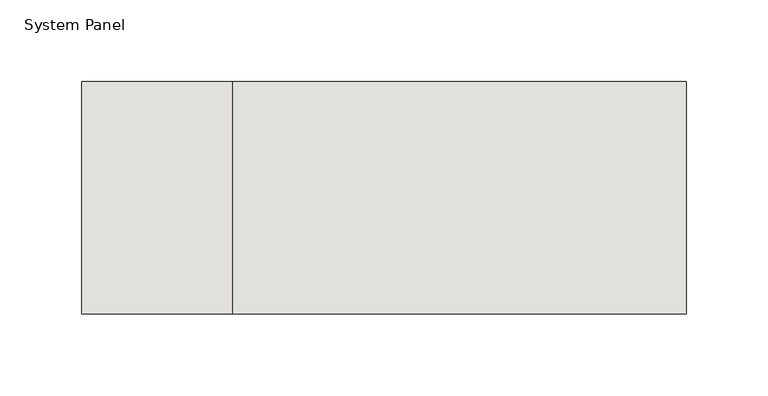
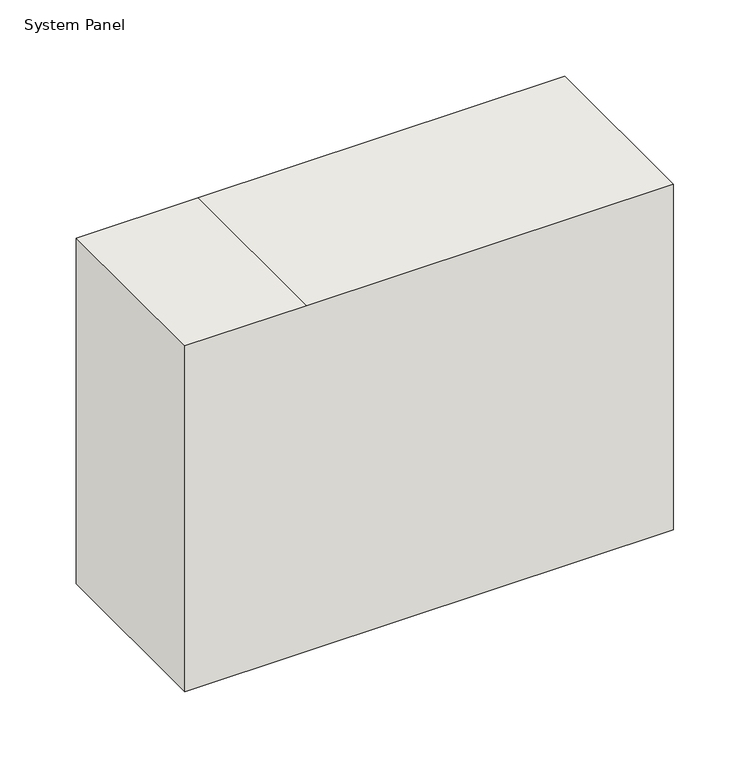
"""IFC4 building model written with IfcOpenShell, lengths in millimetres: wall geometry, System Panel : NLRS_21_CWP_hsb-vulling minerale wol 142 _gen_rsf."""

from ifc_helpers import new_model, si_unit, frame, origin, place, context, project, spatial, polyline, outline, extrude, source, transform, mapped, element, save


def system_panel_b83392b1(model_context):
    return source(origin(), model_context, "Body", "SweptSolid", [
        extrude(outline(polyline([(0.0, -184.5), (0.0, -92.5), (0.0, 184.5), (276.0, 184.5), (276.0, -92.5), (276.0, -184.5), (0.0, -184.5)])), frame((0.0, -71.0, 0.0), z_axis=(0.0, 1.0, 0.0), x_axis=(0.0, 0.0, 1.0)), (0.0, 0.0, 1.0), 142.0),
    ])


if __name__ == "__main__":
    model = new_model("IFC4")
    model_context = context("Model", 3, world=origin())
    ifc_project = project(units=[si_unit("LENGTHUNIT", "METRE", prefix="MILLI")], contexts=[model_context])
    site = spatial("IfcSite", under=ifc_project)
    building = spatial("IfcBuilding", under=site)
    placement = place(None, origin())
    system_panel_shape = system_panel_b83392b1(model_context)
    element("IfcWall", 1, ObjectType="System Panel : NLRS_21_CWP_hsb-vulling minerale wol 142 _gen_rsf", at=placement, inside=building, context=model_context, shape_type="MappedRepresentation", body=[
        mapped(system_panel_shape, transform((0.0, 0.0, 0.0), x_axis=(1.0, 0.0, 0.0), y_axis=(0.0, 1.0, 0.0), z_axis=(0.0, 0.0, 1.0))),
    ])
    save(model, "model.ifc")

# Revit data of these elements
# Type "System Panel : NLRS_21_CWP_hsb-vulling minerale wol 142 _gen_rsf"
#   Type IfcGUID = "07M7mRoiH1CR8m_RSKIwpC"
#   Assembly Code = "21.23"
#   IfcExportAs = "IfcWall"
# Element 1 (IfcWall, "System Panel : NLRS_21_CWP_hsb-vulling minerale wol 142 _gen_rsf")
#   Materials on its faces: "NLRS_m1_isolatie minerale wol_gen_rsf"
# Materials
#   "NLRS_m1_isolatie minerale wol_gen_rsf": class "M - Anorganische materialen", colour RGB 200 200 140, transparency 0, Keynote = "m1", Manufacturer = "Revit Standards Foundation", URL = "www.revitstandards.org", Description = "isolatie minerale wol", Cost = 0
